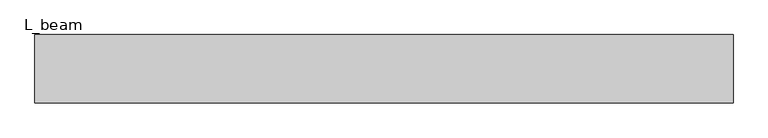
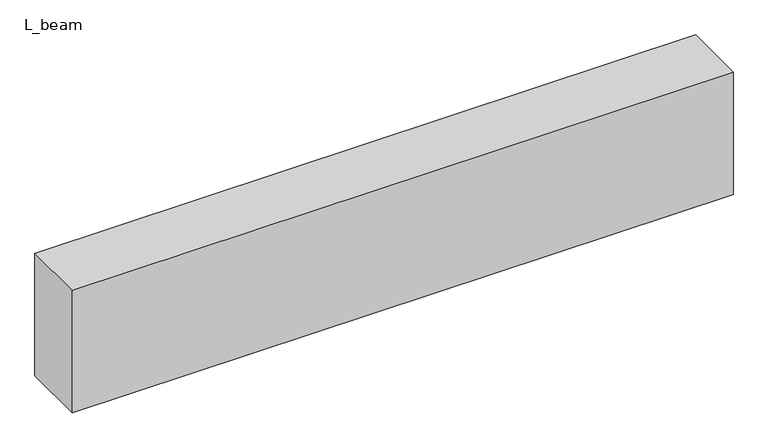
"""IFC4 building model written with IfcOpenShell, lengths in millimetres: beam geometry, 混凝土 - 矩形梁 : L_beam."""

from ifc_helpers import new_model, si_unit, frame, origin, place, context, project, spatial, polyline, outline, extrude, source, transform, mapped, element, save


def l_beam_55392dd8(model_context):
    return source(origin(), model_context, "Body", "SweptSolid", [
        extrude(outline(polyline([(1530.0, 150.0), (1530.0, -150.0), (-1530.0, -150.0), (-1530.0, 150.0), (1530.0, 150.0)])), frame((0.0, 0.0, -300.0), z_axis=(0.0, 0.0, 1.0), x_axis=(1.0, 0.0, 0.0)), (0.0, 0.0, 1.0), 600.0),
    ])


if __name__ == "__main__":
    model = new_model("IFC4")
    model_context = context("Model", 3, world=origin())
    ifc_project = project(units=[si_unit("LENGTHUNIT", "METRE", prefix="MILLI")], contexts=[model_context])
    site = spatial("IfcSite", under=ifc_project)
    building = spatial("IfcBuilding", under=site)
    placement = place(None, origin())
    l_beam_shape = l_beam_55392dd8(model_context)
    element("IfcBeam", 1, ObjectType="混凝土 - 矩形梁 : L_beam", at=placement, inside=building, context=model_context, shape_type="MappedRepresentation", body=[
        mapped(l_beam_shape, transform((0.0, 0.0, 0.0), x_axis=(1.0, 0.0, 0.0), y_axis=(0.0, 1.0, 0.0), z_axis=(0.0, 0.0, 1.0))),
    ])
    save(model, "model.ifc")

# Revit data of these elements
# Type "混凝土 - 矩形梁 : L_beam"
#   Length [instance default] = 1524 mm
#   b = 300 mm
#   h = 600 mm
#   Structural Material [instance default] = none
#   Assembly Code = ""
